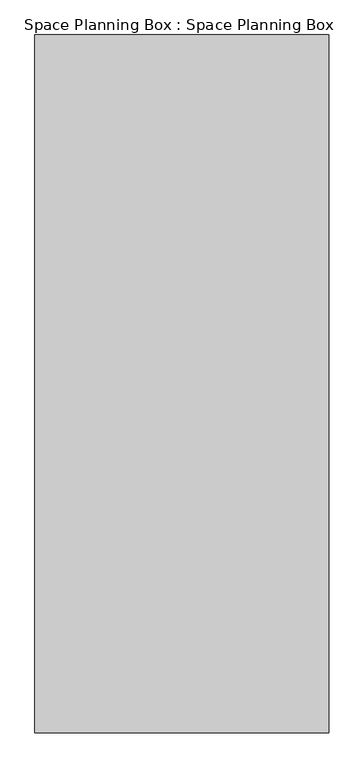
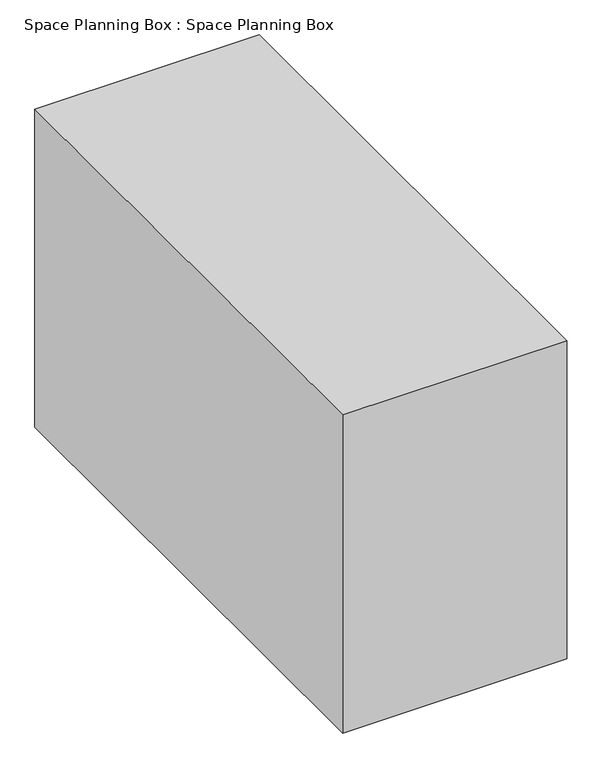
"""IFC4 building model written with IfcOpenShell, lengths in millimetres: proxy geometry, Space Planning Box : Space Planning Box."""

from ifc_helpers import new_model, si_unit, origin, origin_with_axes, place, context, project, spatial, polyline, outline, extrude, source, transform, mapped, element, save


def space_planning_box_space_planning_box_3a820573(model_context):
    return source(origin(), model_context, "Body", "SweptSolid", [
        extrude(outline(polyline([(2000.0, 4750.0), (2000.0, -4750.0), (-2000.0, -4750.0), (-2000.0, 4750.0), (2000.0, 4750.0)])), origin_with_axes(), (0.0, 0.0, 1.0), 6000.0),
    ])


if __name__ == "__main__":
    model = new_model("IFC4")
    model_context = context("Model", 3, world=origin())
    ifc_project = project(units=[si_unit("LENGTHUNIT", "METRE", prefix="MILLI")], contexts=[model_context])
    site = spatial("IfcSite", under=ifc_project)
    building = spatial("IfcBuilding", under=site)
    placement = place(None, origin())
    space_planning_box_space_planning_box_shape = space_planning_box_space_planning_box_3a820573(model_context)
    element("IfcBuildingElementProxy", 1, Name="Space Planning Box : Space Planning Box", ObjectType="Space Planning Box : Space Planning Box", at=placement, inside=building, context=model_context, shape_type="MappedRepresentation", body=[
        mapped(space_planning_box_space_planning_box_shape, transform((0.0, 0.0, 0.0), x_axis=(1.0, 0.0, 0.0), y_axis=(0.0, 1.0, 0.0), z_axis=(0.0, 0.0, 1.0))),
    ])
    save(model, "model.ifc")

# Revit data of these elements
# Type "Space Planning Box : Space Planning Box"
#   Type Comments = "..."
#   Room Name [instance default] = "?"
#   Assembly Code = "..."
#   Width [instance default] = 1524 mm
#   Program Area [instance default] = 0 m²
#   Length [instance default] = 1524 mm
#   Height [instance default] = 1524 mm
#   Area [instance default] = 2.32258 m²
#   Fill Color [instance default] = Cyan
#   Default Elevation = 0
# Element 1 (IfcBuildingElementProxy, "Space Planning Box : Space Planning Box")
#   Room Name = "Stairway"
#   Width = 4000 mm
#   Program Area = 38 m²
#   Length = 9500 mm
#   Height = 6000 mm
#   Area = 38 m²
#   Fill Color = Lavender
#   Materials on its faces: "Lavender"
# Materials
#   "Cyan": class "Generic", colour RGB 0 255 255, transparency 0.2, Cost = 0
#   "Lavender": class "Generic", colour RGB 186 85 211, transparency 0.2, Cost = 0
